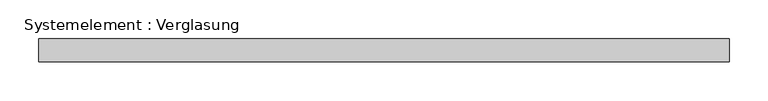
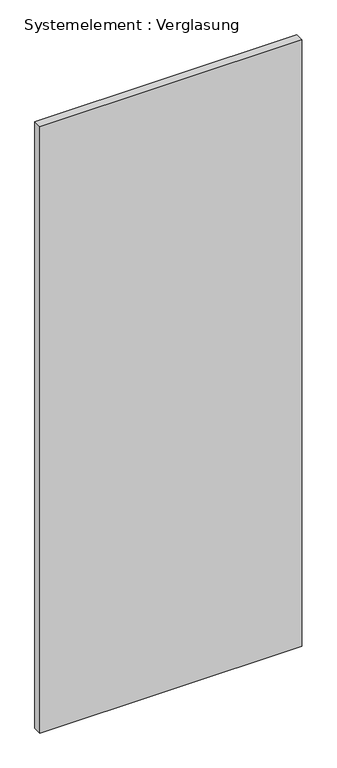
"""IFC4 building model written with IfcOpenShell, lengths in millimetres: plate geometry, Systemelement : Verglasung."""

from ifc_helpers import new_model, si_unit, origin, origin_with_axes, place, context, project, spatial, polyline, outline, extrude, source, transform, mapped, element, save


def systemelement_verglasung_9de6bae2(model_context):
    return source(origin(), model_context, "Body", "SweptSolid", [
        extrude(outline(polyline([(447.5113473, -15.0), (-447.5113473, -15.0), (-447.5113473, 15.0), (447.5113473, 15.0), (447.5113473, -15.0)])), origin_with_axes(), (0.0, 0.0, 1.0), 2190.0),
    ])


if __name__ == "__main__":
    model = new_model("IFC4")
    model_context = context("Model", 3, world=origin())
    ifc_project = project(units=[si_unit("LENGTHUNIT", "METRE", prefix="MILLI")], contexts=[model_context])
    site = spatial("IfcSite", under=ifc_project)
    building = spatial("IfcBuilding", under=site)
    placement = place(None, origin())
    systemelement_verglasung_shape = systemelement_verglasung_9de6bae2(model_context)
    element("IfcPlate", 1, ObjectType="Systemelement : Verglasung", at=placement, inside=building, context=model_context, shape_type="MappedRepresentation", body=[
        mapped(systemelement_verglasung_shape, transform((0.0, 0.0, 0.0), x_axis=(1.0, 0.0, 0.0), y_axis=(0.0, 1.0, 0.0), z_axis=(0.0, 0.0, 1.0))),
    ])
    save(model, "model.ifc")

# Revit data of these elements
# Type "Systemelement : Verglasung"
#   Construction Type Id = "GSP4R"
#   Analytic Construction = "1/8 Zoll Pilkington-Verglasung einfach"
#   Visual Light Transmittance = 0.9
#   Solar Heat Gain Coefficient = 0.86
#   Heat Transfer Coefficient (U) = 6.7069 W/(m²·K)
# Element 1 (IfcPlate, "Systemelement : Verglasung")
#   Materials on its faces: "Glas"
# Materials
#   "Glas": class "Glas", colour RGB 0 0 255, transparency 0.75, Comments = "Render-Darstellung nicht aktualisiert ", Cost = 0
